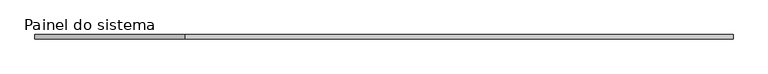
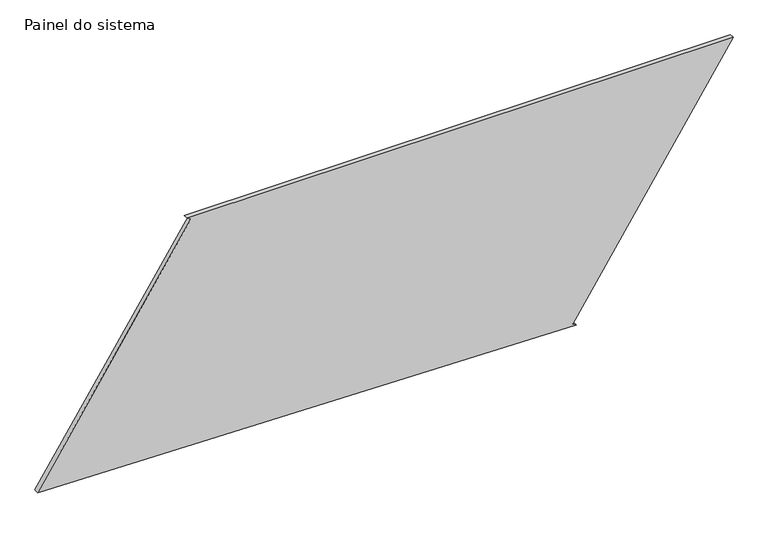
"""IFC4 building model written with IfcOpenShell, lengths in millimetres: plate geometry, Painel do sistema : Envidraçado."""

import ifcopenshell
import ifcopenshell.guid

model = None  # the IFC model being written
_history = None  # IfcOwnerHistory: only IFC2X3 demands one
_inside = {}  # id of a spatial element -> (the spatial element, [elements in it])
_under = {}  # id of a project, library or spatial element -> (it, [spatial elements below it])
_declared = {}  # id of a project -> (the project, [libraries it declares])
_typed = {}  # id of a type object -> (the type object, [elements of that type])
_made_of = {}  # id of a material, layer set ... -> (it, [elements and type objects made of it])


def new_model(schema):
    """Start an empty IFC model of exactly this schema.

    Asked for "IFC4X3", IfcOpenShell would pick the latest addendum, in which some entities
    have other attributes; the version numbers below select the first issue.
    IFC2X3 requires an IfcOwnerHistory on every rooted entity: one is made here for all.
    """
    global model, _history
    if schema == "IFC4X3":
        model = ifcopenshell.file(schema_version=(4, 3, 0, 0))
    else:
        model = ifcopenshell.file(schema=schema)
    _inside.clear()
    _under.clear()
    _declared.clear()
    _typed.clear()
    _made_of.clear()
    _history = None
    if model.schema == "IFC2X3":
        org = make("IfcOrganization", Name="unknown")
        user = make(
            "IfcPersonAndOrganization",
            ThePerson=make("IfcPerson", FamilyName="unknown"),
            TheOrganization=org,
        )
        app = make(
            "IfcApplication",
            ApplicationDeveloper=org,
            Version="unknown",
            ApplicationFullName="unknown",
            ApplicationIdentifier="unknown",
        )
        _history = make(
            "IfcOwnerHistory",
            OwningUser=user,
            OwningApplication=app,
            ChangeAction="ADDED",
            CreationDate=0,
        )
    return model


def make(cls, **values):
    """One entity of the class cls with the attributes given. An attribute that is None is left unset."""
    return model.create_entity(
        cls, **{name: value for name, value in values.items() if value is not None}
    )


def rooted(cls, **values):
    """An entity with a GlobalId (a new one), such as an element, a storey or a relation."""
    return make(cls, GlobalId=ifcopenshell.guid.new(), OwnerHistory=_history, **values)


def si_unit(unit_type, name, prefix=None):
    """IfcSIUnit, for example si_unit("LENGTHUNIT", "METRE", prefix="MILLI")."""
    return make("IfcSIUnit", UnitType=unit_type, Prefix=prefix, Name=name)


def assignment(units):
    """IfcUnitAssignment: the units of a project."""
    return None if units is None else make("IfcUnitAssignment", Units=units)


def point(xyz):
    """IfcCartesianPoint."""
    return None if xyz is None else make("IfcCartesianPoint", Coordinates=xyz)


def direction(xyz):
    """IfcDirection."""
    return None if xyz is None else make("IfcDirection", DirectionRatios=xyz)


def frame(location, z_axis=None, x_axis=None):
    """IfcAxis2Placement3D, a coordinate frame: its origin and axes. An axis left out is left unset."""
    return make(
        "IfcAxis2Placement3D",
        Location=point(location),
        Axis=direction(z_axis),
        RefDirection=direction(x_axis),
    )


def origin():
    """The frame at (0, 0, 0) with its axes left unset."""
    return frame((0.0, 0.0, 0.0))


def place(relative_to, where):
    """IfcLocalPlacement: puts the frame where relative to a parent placement (None: the world)."""
    return make(
        "IfcLocalPlacement", PlacementRelTo=relative_to, RelativePlacement=where
    )


def context(
    kind, dimensions, precision=None, world=None, true_north=None, identifier=None
):
    """IfcGeometricRepresentationContext, for example the 3D "Model" context."""
    return make(
        "IfcGeometricRepresentationContext",
        ContextIdentifier=identifier,
        ContextType=kind,
        CoordinateSpaceDimension=dimensions,
        Precision=precision,
        WorldCoordinateSystem=world,
        TrueNorth=true_north,
    )


def project(units=None, contexts=None):
    """IfcProject with its units and contexts."""
    return rooted(
        "IfcProject",
        Name="project",
        RepresentationContexts=contexts,
        UnitsInContext=assignment(units),
    )


def spatial(cls, under=None, at=None, **own):
    """A site, building, storey or space (cls), placed at a placement, below another one or the project."""
    s = rooted(cls, ObjectPlacement=at, **own)
    if under is not None:
        _under.setdefault(under.id(), (under, []))[1].append(s)
    return s


def polyline(points):
    """IfcPolyline through the points."""
    return make("IfcPolyline", Points=[point(p) for p in points])


def outline(outer, holes=None, kind="AREA"):
    """IfcArbitraryClosedProfileDef: a profile drawn as a closed curve; with holes, ...WithVoids."""
    if holes is None:
        return make("IfcArbitraryClosedProfileDef", ProfileType=kind, OuterCurve=outer)
    return make(
        "IfcArbitraryProfileDefWithVoids",
        ProfileType=kind,
        OuterCurve=outer,
        InnerCurves=holes,
    )


def extrude(swept, where, along, depth):
    """IfcExtrudedAreaSolid: the profile swept, set in the frame where, extruded along a direction by depth."""
    return make(
        "IfcExtrudedAreaSolid",
        SweptArea=swept,
        Position=where,
        ExtrudedDirection=direction(along),
        Depth=depth,
    )


def shape(context_of_items, identifier, shape_type, items):
    """IfcShapeRepresentation: the items that make up one representation, for example the "Body"."""
    return make(
        "IfcShapeRepresentation",
        ContextOfItems=context_of_items,
        RepresentationIdentifier=identifier,
        RepresentationType=shape_type,
        Items=items,
    )


def source(mapping_origin, context_of_items, identifier, shape_type, items):
    """IfcRepresentationMap: a shape defined once, which mapped items show again and again."""
    return make(
        "IfcRepresentationMap",
        MappingOrigin=mapping_origin,
        MappedRepresentation=shape(context_of_items, identifier, shape_type, items),
    )


def transform(
    local_origin,
    x_axis=None,
    y_axis=None,
    z_axis=None,
    scale=None,
    scale2=None,
    scale3=None,
    uniform=True,
):
    """IfcCartesianTransformationOperator3D, or its non-uniform kind. x_axis, y_axis, z_axis: its Axis1, 2, 3."""
    if uniform:
        return make(
            "IfcCartesianTransformationOperator3D",
            Axis1=direction(x_axis),
            Axis2=direction(y_axis),
            LocalOrigin=point(local_origin),
            Scale=scale,
            Axis3=direction(z_axis),
        )
    return make(
        "IfcCartesianTransformationOperator3DnonUniform",
        Axis1=direction(x_axis),
        Axis2=direction(y_axis),
        LocalOrigin=point(local_origin),
        Scale=scale,
        Axis3=direction(z_axis),
        Scale2=scale2,
        Scale3=scale3,
    )


def mapped(mapping_source, mapping_target):
    """IfcMappedItem: shows the shape of a source again, moved by a transform."""
    return make(
        "IfcMappedItem", MappingSource=mapping_source, MappingTarget=mapping_target
    )


def made_of(thing, what):
    """Note that an element or type object is made of a material, layer set ...; save() writes the relation."""
    if what is not None:
        _made_of.setdefault(what.id(), (what, []))[1].append(thing)
    return thing


def element(
    cls,
    number,
    at=None,
    inside=None,
    cuts=None,
    type_object=None,
    material=None,
    context=None,
    identifier="Body",
    shape_type=None,
    held_by="IfcProductDefinitionShape",
    body=None,
    shapes=None,
    **own,
):
    """One element of the class cls, such as IfcWall. Its Tag is "e" and its number.

    at: its placement. inside: the storey or other place that contains it. cuts: it is an
    opening in that element (IfcRelVoidsElement). A single representation is given by context,
    identifier, shape_type and body (its items); several are given by shapes. held_by: the class
    of the entity that holds the representations. save() writes the other relations.
    """
    e = rooted(cls, Tag="e%d" % number, ObjectPlacement=at, **own)
    if body is not None:
        shapes = [shape(context, identifier, shape_type, body)]
    if shapes is not None:
        e.Representation = make(held_by, Representations=shapes)
    if inside is not None:
        _inside.setdefault(inside.id(), (inside, []))[1].append(e)
    if cuts is not None:
        rooted(
            "IfcRelVoidsElement", RelatingBuildingElement=cuts, RelatedOpeningElement=e
        )
    if type_object is not None:
        _typed.setdefault(type_object.id(), (type_object, []))[1].append(e)
    return made_of(e, material)


def aggregate(whole, parts):
    """IfcRelAggregates: a whole, such as a stair, and the parts it consists of."""
    return rooted("IfcRelAggregates", RelatingObject=whole, RelatedObjects=parts)


def save(model, path):
    """Write the relations noted so far, then the file.

    IfcRelAggregates (storeys below a building ...), IfcRelContainedInSpatialStructure (elements
    in a storey), IfcRelDefinesByType, IfcRelAssociatesMaterial and IfcRelDeclares: one each for
    every whole, place, type object, material and project.
    """
    for whole, parts in _under.values():
        aggregate(whole, parts)
    for where, things in _inside.values():
        rooted(
            "IfcRelContainedInSpatialStructure",
            RelatedElements=things,
            RelatingStructure=where,
        )
    for kind, things in _typed.values():
        rooted("IfcRelDefinesByType", RelatedObjects=things, RelatingType=kind)
    for what, things in _made_of.values():
        rooted("IfcRelAssociatesMaterial", RelatedObjects=things, RelatingMaterial=what)
    for by, libraries in _declared.values():
        rooted("IfcRelDeclares", RelatingContext=by, RelatedDefinitions=libraries)
    model.write(path)


def painel_do_sistema_e3a05b94(model_context):
    return source(origin(), model_context, "Body", "SweptSolid", [
        extrude(outline(polyline([(0.0, 1063.2811638), (13.6354654, 1042.3270692), (1387.1343062, 1936.1044538), (1387.1343062, -1103.4314686), (1373.4988407, -1082.4773739), (61.7003719, -1936.1044538), (0.0, 1063.2811638)])), frame((0.0, 24.5, 0.0), z_axis=(0.0, 1.0, 0.0), x_axis=(0.0, 0.0, 1.0)), (0.0, 0.0, 1.0), 25.0),
    ])


if __name__ == "__main__":
    model = new_model("IFC4")
    model_context = context("Model", 3, world=origin())
    ifc_project = project(units=[si_unit("LENGTHUNIT", "METRE", prefix="MILLI")], contexts=[model_context])
    site = spatial("IfcSite", under=ifc_project)
    building = spatial("IfcBuilding", under=site)
    placement = place(None, origin())
    painel_do_sistema_shape = painel_do_sistema_e3a05b94(model_context)
    element("IfcPlate", 1, ObjectType="Painel do sistema : Envidraçado", at=placement, inside=building, context=model_context, shape_type="MappedRepresentation", body=[
        mapped(painel_do_sistema_shape, transform((0.0, 0.0, 0.0), x_axis=(1.0, 0.0, 0.0), y_axis=(0.0, 1.0, 0.0), z_axis=(0.0, 0.0, 1.0))),
    ])
    save(model, "model.ifc")

# Revit data of these elements
# Type "Painel do sistema : Envidraçado"
#   Construction Type Id = "GSP4R"
#   Analytic Construction = "Vidraça única Pilkington 1/8 pol"
#   Visual Light Transmittance = 0.9
#   Solar Heat Gain Coefficient = 0.86
#   Heat Transfer Coefficient (U) = 6.7069 W/(m²·K)
# Element 1 (IfcPlate, "Painel do sistema : Envidraçado")
#   Materials on its faces: "Vidro"
# Materials
#   "Vidro": class "Vidro", colour RGB 0 128 192, transparency 0.9, Description = "Vidro de sílica", Cost = 0
